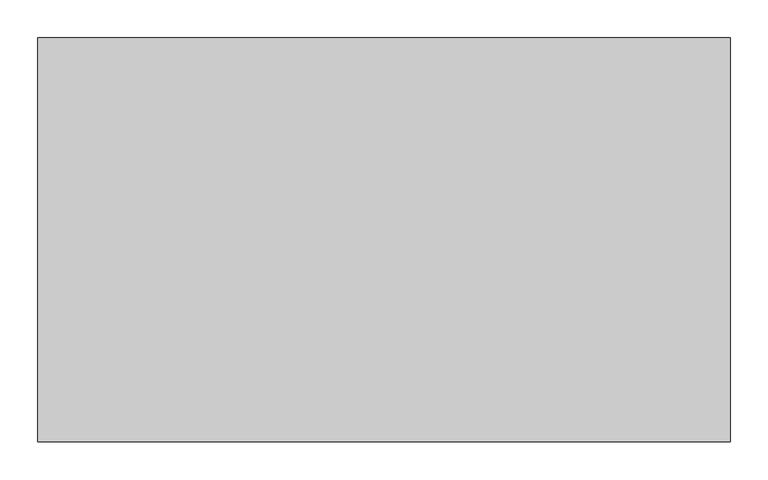
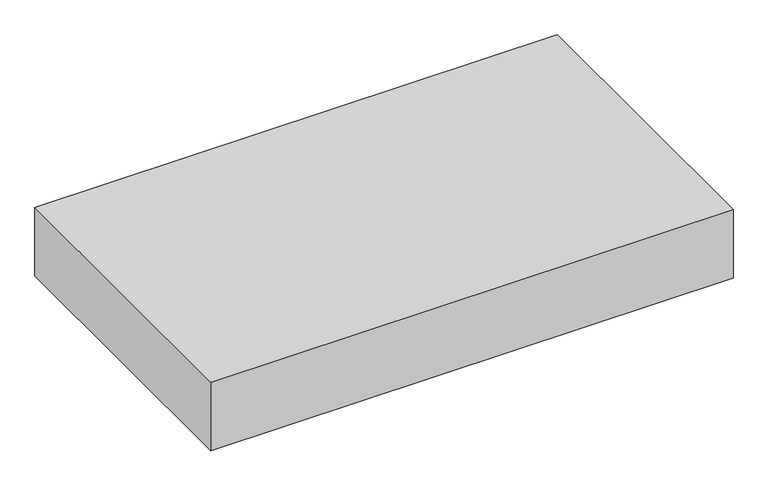
"""IFC4 building model written with IfcOpenShell, lengths in millimetres: proxy geometry, A4995 - Table, Diaper Changing, Wall Mounted : A4995 - Table, Diaper Changing, Wall Mounted."""

import ifcopenshell
import ifcopenshell.guid

model = None  # the IFC model being written
_history = None  # IfcOwnerHistory: only IFC2X3 demands one
_inside = {}  # id of a spatial element -> (the spatial element, [elements in it])
_under = {}  # id of a project, library or spatial element -> (it, [spatial elements below it])
_declared = {}  # id of a project -> (the project, [libraries it declares])
_typed = {}  # id of a type object -> (the type object, [elements of that type])
_made_of = {}  # id of a material, layer set ... -> (it, [elements and type objects made of it])


def new_model(schema):
    """Start an empty IFC model of exactly this schema.

    Asked for "IFC4X3", IfcOpenShell would pick the latest addendum, in which some entities
    have other attributes; the version numbers below select the first issue.
    IFC2X3 requires an IfcOwnerHistory on every rooted entity: one is made here for all.
    """
    global model, _history
    if schema == "IFC4X3":
        model = ifcopenshell.file(schema_version=(4, 3, 0, 0))
    else:
        model = ifcopenshell.file(schema=schema)
    _inside.clear()
    _under.clear()
    _declared.clear()
    _typed.clear()
    _made_of.clear()
    _history = None
    if model.schema == "IFC2X3":
        org = make("IfcOrganization", Name="unknown")
        user = make(
            "IfcPersonAndOrganization",
            ThePerson=make("IfcPerson", FamilyName="unknown"),
            TheOrganization=org,
        )
        app = make(
            "IfcApplication",
            ApplicationDeveloper=org,
            Version="unknown",
            ApplicationFullName="unknown",
            ApplicationIdentifier="unknown",
        )
        _history = make(
            "IfcOwnerHistory",
            OwningUser=user,
            OwningApplication=app,
            ChangeAction="ADDED",
            CreationDate=0,
        )
    return model


def make(cls, **values):
    """One entity of the class cls with the attributes given. An attribute that is None is left unset."""
    return model.create_entity(
        cls, **{name: value for name, value in values.items() if value is not None}
    )


def rooted(cls, **values):
    """An entity with a GlobalId (a new one), such as an element, a storey or a relation."""
    return make(cls, GlobalId=ifcopenshell.guid.new(), OwnerHistory=_history, **values)


def si_unit(unit_type, name, prefix=None):
    """IfcSIUnit, for example si_unit("LENGTHUNIT", "METRE", prefix="MILLI")."""
    return make("IfcSIUnit", UnitType=unit_type, Prefix=prefix, Name=name)


def assignment(units):
    """IfcUnitAssignment: the units of a project."""
    return None if units is None else make("IfcUnitAssignment", Units=units)


def point(xyz):
    """IfcCartesianPoint."""
    return None if xyz is None else make("IfcCartesianPoint", Coordinates=xyz)


def direction(xyz):
    """IfcDirection."""
    return None if xyz is None else make("IfcDirection", DirectionRatios=xyz)


def frame(location, z_axis=None, x_axis=None):
    """IfcAxis2Placement3D, a coordinate frame: its origin and axes. An axis left out is left unset."""
    return make(
        "IfcAxis2Placement3D",
        Location=point(location),
        Axis=direction(z_axis),
        RefDirection=direction(x_axis),
    )


def origin():
    """The frame at (0, 0, 0) with its axes left unset."""
    return frame((0.0, 0.0, 0.0))


def origin_with_axes():
    """The frame at (0, 0, 0) with the z axis (0, 0, 1) and the x axis (1, 0, 0) written out."""
    return frame((0.0, 0.0, 0.0), z_axis=(0.0, 0.0, 1.0), x_axis=(1.0, 0.0, 0.0))


def place(relative_to, where):
    """IfcLocalPlacement: puts the frame where relative to a parent placement (None: the world)."""
    return make(
        "IfcLocalPlacement", PlacementRelTo=relative_to, RelativePlacement=where
    )


def context(
    kind, dimensions, precision=None, world=None, true_north=None, identifier=None
):
    """IfcGeometricRepresentationContext, for example the 3D "Model" context."""
    return make(
        "IfcGeometricRepresentationContext",
        ContextIdentifier=identifier,
        ContextType=kind,
        CoordinateSpaceDimension=dimensions,
        Precision=precision,
        WorldCoordinateSystem=world,
        TrueNorth=true_north,
    )


def project(units=None, contexts=None):
    """IfcProject with its units and contexts."""
    return rooted(
        "IfcProject",
        Name="project",
        RepresentationContexts=contexts,
        UnitsInContext=assignment(units),
    )


def spatial(cls, under=None, at=None, **own):
    """A site, building, storey or space (cls), placed at a placement, below another one or the project."""
    s = rooted(cls, ObjectPlacement=at, **own)
    if under is not None:
        _under.setdefault(under.id(), (under, []))[1].append(s)
    return s


def polyline(points):
    """IfcPolyline through the points."""
    return make("IfcPolyline", Points=[point(p) for p in points])


def outline(outer, holes=None, kind="AREA"):
    """IfcArbitraryClosedProfileDef: a profile drawn as a closed curve; with holes, ...WithVoids."""
    if holes is None:
        return make("IfcArbitraryClosedProfileDef", ProfileType=kind, OuterCurve=outer)
    return make(
        "IfcArbitraryProfileDefWithVoids",
        ProfileType=kind,
        OuterCurve=outer,
        InnerCurves=holes,
    )


def extrude(swept, where, along, depth):
    """IfcExtrudedAreaSolid: the profile swept, set in the frame where, extruded along a direction by depth."""
    return make(
        "IfcExtrudedAreaSolid",
        SweptArea=swept,
        Position=where,
        ExtrudedDirection=direction(along),
        Depth=depth,
    )


def shape(context_of_items, identifier, shape_type, items):
    """IfcShapeRepresentation: the items that make up one representation, for example the "Body"."""
    return make(
        "IfcShapeRepresentation",
        ContextOfItems=context_of_items,
        RepresentationIdentifier=identifier,
        RepresentationType=shape_type,
        Items=items,
    )


def source(mapping_origin, context_of_items, identifier, shape_type, items):
    """IfcRepresentationMap: a shape defined once, which mapped items show again and again."""
    return make(
        "IfcRepresentationMap",
        MappingOrigin=mapping_origin,
        MappedRepresentation=shape(context_of_items, identifier, shape_type, items),
    )


def transform(
    local_origin,
    x_axis=None,
    y_axis=None,
    z_axis=None,
    scale=None,
    scale2=None,
    scale3=None,
    uniform=True,
):
    """IfcCartesianTransformationOperator3D, or its non-uniform kind. x_axis, y_axis, z_axis: its Axis1, 2, 3."""
    if uniform:
        return make(
            "IfcCartesianTransformationOperator3D",
            Axis1=direction(x_axis),
            Axis2=direction(y_axis),
            LocalOrigin=point(local_origin),
            Scale=scale,
            Axis3=direction(z_axis),
        )
    return make(
        "IfcCartesianTransformationOperator3DnonUniform",
        Axis1=direction(x_axis),
        Axis2=direction(y_axis),
        LocalOrigin=point(local_origin),
        Scale=scale,
        Axis3=direction(z_axis),
        Scale2=scale2,
        Scale3=scale3,
    )


def mapped(mapping_source, mapping_target):
    """IfcMappedItem: shows the shape of a source again, moved by a transform."""
    return make(
        "IfcMappedItem", MappingSource=mapping_source, MappingTarget=mapping_target
    )


def made_of(thing, what):
    """Note that an element or type object is made of a material, layer set ...; save() writes the relation."""
    if what is not None:
        _made_of.setdefault(what.id(), (what, []))[1].append(thing)
    return thing


def element(
    cls,
    number,
    at=None,
    inside=None,
    cuts=None,
    type_object=None,
    material=None,
    context=None,
    identifier="Body",
    shape_type=None,
    held_by="IfcProductDefinitionShape",
    body=None,
    shapes=None,
    **own,
):
    """One element of the class cls, such as IfcWall. Its Tag is "e" and its number.

    at: its placement. inside: the storey or other place that contains it. cuts: it is an
    opening in that element (IfcRelVoidsElement). A single representation is given by context,
    identifier, shape_type and body (its items); several are given by shapes. held_by: the class
    of the entity that holds the representations. save() writes the other relations.
    """
    e = rooted(cls, Tag="e%d" % number, ObjectPlacement=at, **own)
    if body is not None:
        shapes = [shape(context, identifier, shape_type, body)]
    if shapes is not None:
        e.Representation = make(held_by, Representations=shapes)
    if inside is not None:
        _inside.setdefault(inside.id(), (inside, []))[1].append(e)
    if cuts is not None:
        rooted(
            "IfcRelVoidsElement", RelatingBuildingElement=cuts, RelatedOpeningElement=e
        )
    if type_object is not None:
        _typed.setdefault(type_object.id(), (type_object, []))[1].append(e)
    return made_of(e, material)


def aggregate(whole, parts):
    """IfcRelAggregates: a whole, such as a stair, and the parts it consists of."""
    return rooted("IfcRelAggregates", RelatingObject=whole, RelatedObjects=parts)


def save(model, path):
    """Write the relations noted so far, then the file.

    IfcRelAggregates (storeys below a building ...), IfcRelContainedInSpatialStructure (elements
    in a storey), IfcRelDefinesByType, IfcRelAssociatesMaterial and IfcRelDeclares: one each for
    every whole, place, type object, material and project.
    """
    for whole, parts in _under.values():
        aggregate(whole, parts)
    for where, things in _inside.values():
        rooted(
            "IfcRelContainedInSpatialStructure",
            RelatedElements=things,
            RelatingStructure=where,
        )
    for kind, things in _typed.values():
        rooted("IfcRelDefinesByType", RelatedObjects=things, RelatingType=kind)
    for what, things in _made_of.values():
        rooted("IfcRelAssociatesMaterial", RelatedObjects=things, RelatingMaterial=what)
    for by, libraries in _declared.values():
        rooted("IfcRelDeclares", RelatingContext=by, RelatedDefinitions=libraries)
    model.write(path)


def specialty_equipment_ed87bb6a(model_context):
    return source(origin(), model_context, "Body", "SweptSolid", [
        extrude(outline(polyline([(457.2, 0.0), (-457.2, 0.0), (-457.2, 533.4), (457.2, 533.4), (457.2, 0.0)])), origin_with_axes(), (0.0, 0.0, 1.0), 127.0),
        extrude(outline(polyline([(457.2, 0.0), (-457.2, 0.0), (-457.2, 533.4), (457.2, 533.4), (457.2, 0.0)])), origin_with_axes(), (0.0, 0.0, 1.0), 127.0),
    ])


if __name__ == "__main__":
    model = new_model("IFC4")
    model_context = context("Model", 3, world=origin())
    ifc_project = project(units=[si_unit("LENGTHUNIT", "METRE", prefix="MILLI")], contexts=[model_context])
    site = spatial("IfcSite", under=ifc_project)
    building = spatial("IfcBuilding", under=site)
    placement = place(None, origin())
    specialty_equipment_shape = specialty_equipment_ed87bb6a(model_context)
    element("IfcBuildingElementProxy", 1, Name="A4995 - Table, Diaper Changing, Wall Mounted : A4995 - Table, Diaper Changing, Wall Mounted", ObjectType="A4995 - Table, Diaper Changing, Wall Mounted : A4995 - Table, Diaper Changing, Wall Mounted", at=placement, inside=building, context=model_context, shape_type="MappedRepresentation", body=[
        mapped(specialty_equipment_shape, transform((0.0, 0.0, 0.0), x_axis=(1.0, 0.0, 0.0), y_axis=(0.0, 1.0, 0.0), z_axis=(0.0, 0.0, 1.0))),
    ])
    save(model, "model.ifc")

# Revit data of these elements
# Type "A4995 - Table, Diaper Changing, Wall Mounted : A4995 - Table, Diaper Changing, Wall Mounted"
#   Watts2 = "0"
#   Watts1 = "0"
#   Unit_Issue = "EA"
#   UTIL_6_Misc = "-"
#   UTIL_5_NonMedGas = "-"
#   UTIL_4_MiscGas = "-"
#   UTIL_3_MedGas = "-"
#   UTIL_2_Elec = "-"
#   UTIL_1_WaterDrain = "-"
#   Nomenclature = "Table, Diaper Changing, Wall Mounted"
#   NSN = "7100"
#   Location [instance default] = ""
#   JSN = "A4995"
#   Fund_Source_VA = "-"
#   Fund_Source_Navy = "-"
#   Fund_Source_Army = "-"
#   Fund_Source_AF = "-"
#   ELEC_Volts2 = "0"
#   ELEC_Volts1 = "0"
#   ELEC_Phase2 = "0"
#   ELEC_Phase1 = "0"
#   ELEC_HertzSwitch = "0"
#   ELEC_HertzDependent = "0"
#   ELEC_Hertz = "0"
#   ELEC_Amps2 = "0"
#   ELEC_Amps1 = "0"
#   DetailDescription = "Wall mounted diaper changing table for use in public restrooms. Unit is a fold down system that folds upward when not in use for minimal intrusion into the room. Changing surface is contoured and has safety belt to insure that an infant will not fall from the table. Table is designed to hold no less than 250 pounds static weight. Closed dimensions are approximately 21\" H x 36\" W x 5\" D. Open dimensions vary according to style. One system''s open dimensions are 15 \" high, 32\" wide and 19\" deep."
#   CAT_VA = "A"
#   CAT_Navy = "A"
#   CAT_IHS = "-"
#   CAT_Army = "A"
#   CAT_AF = "A"
#   BTUperhour = "0"
#   Weight_IP = 26
#   Default Elevation = 2' - 5"
#   DIM_Width_IP = 3' - 0"
#   DIM_Height_IP = 1' - 9"
#   DIM_Depth_IP = 0' - 5"
#   Assembly Code = ""
# Element 1 (IfcBuildingElementProxy, "A4995 - Table, Diaper Changing, Wall Mounted : A4995 - Table, Diaper Changing, Wall Mounted")
#   Location = "TLTU1"
#   Materials on its faces: "EquipSpace"
# Materials
#   "EquipSpace": class "Unassigned", colour RGB 221 217 195, transparency 0.5
